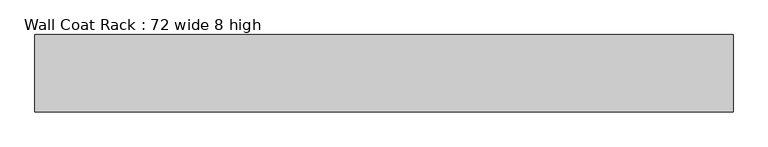
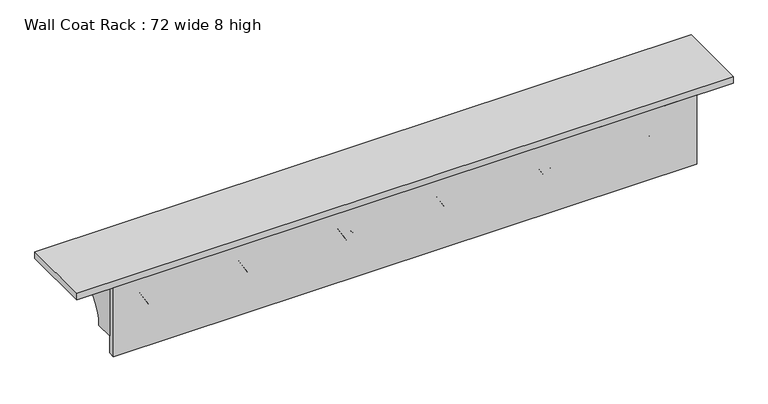
"""IFC4 building model written with IfcOpenShell, lengths in millimetres: furniture geometry, Wall Coat Rack : 72 wide 8 high."""

from ifc_helpers import new_model, si_unit, point, frame, frame_2d, origin, place, context, project, spatial, polyline, circle_curve, ellipse_curve, trimmed, segment, composite_curve, outline, extrude, source, transform, mapped, element, save
from ifc_brep_helpers import plane_surface, revolved_surface, advanced_brep


def wall_coat_rack_72_wide_8_high_2e9e28dd(model_context):
    return source(origin(), model_context, "Body", "SolidModel", [
        advanced_brep(
        [(-419.7046589, 92.075, 1574.8), (-394.3046589, 92.075, 1574.8), (-407.0046589, 92.075, 1574.8), (-419.7046589, 193.675, 1574.8), (-394.3046589, 193.675, 1574.8), (-407.0046589, 193.675, 1574.8)],
        [
            (0, 1, circle_curve(frame((-407.0046589, 92.075, 1574.8), z_axis=(0.0, -1.0, 0.0), x_axis=(1.0, 0.0, 0.0)), 12.7)),
            (1, 2),
            (2, 0),
            (1, 0, circle_curve(frame((-407.0046589, 92.075, 1574.8), z_axis=(0.0, -1.0, 0.0), x_axis=(1.0, 0.0, 0.0)), 12.7)),
            (3, 4, circle_curve(frame((-407.0046589, 193.675, 1574.8), z_axis=(0.0, -1.0, 0.0), x_axis=(1.0, 0.0, 0.0)), 12.7)),
            (4, 1, circle_curve(frame((-119.5616517, 142.875, 1574.8), z_axis=(0.0, 0.0, 1.0), x_axis=(1.0, 0.0, 0.0)), 279.4)),
            (0, 3, circle_curve(frame((-694.4476661, 142.875, 1574.8), z_axis=(0.0, 0.0, 1.0), x_axis=(-1.0, 0.0, 0.0)), 279.4)),
            (4, 3, circle_curve(frame((-407.0046589, 193.675, 1574.8), z_axis=(0.0, -1.0, 0.0), x_axis=(1.0, 0.0, 0.0)), 12.7)),
            (5, 4),
            (3, 5),
        ],
        [
            plane_surface(frame((-407.0046589, 92.075, 1574.8), z_axis=(0.0, -1.0, 0.0), x_axis=(1.0, 0.0, 0.0))),
            revolved_surface(trimmed(ellipse_curve(frame((-119.5616517, 142.875, 1574.8), z_axis=(0.0, 0.0, -1.0), x_axis=(1.0, 0.0, 0.0)), 279.4, 279.4), [point((-394.3046589, 92.075, 1574.8))], [point((-394.3046589, 193.675, 1574.8))], True, "CARTESIAN"), (-407.0046589, 193.675, 1574.8), (0.0, 1.0, 0.0)),
            plane_surface(frame((-407.0046589, 193.675, 1574.8), z_axis=(0.0, 1.0, 0.0), x_axis=(1.0, 0.0, 0.0))),
        ],
        [
            (0, [[1, 2, 3]]),
            (0, [[4, -3, -2]]),
            (1, [[5, 6, -1, 7]]),
            (1, [[8, -7, -4, -6]]),
            (2, [[9, -5, 10]]),
            (2, [[-10, -8, -9]]),
        ],
    ),
        advanced_brep(
        [(-145.3846589, 88.9, 1574.8), (-119.9846589, 88.9, 1574.8), (-132.6846589, 88.9, 1574.8), (-145.3846589, 190.5, 1574.8), (-119.9846589, 190.5, 1574.8), (-132.6846589, 190.5, 1574.8)],
        [
            (0, 1, circle_curve(frame((-132.6846589, 88.9, 1574.8), z_axis=(0.0, -1.0, 0.0), x_axis=(1.0, 0.0, 0.0)), 12.7)),
            (1, 2),
            (2, 0),
            (1, 0, circle_curve(frame((-132.6846589, 88.9, 1574.8), z_axis=(0.0, -1.0, 0.0), x_axis=(1.0, 0.0, 0.0)), 12.7)),
            (3, 4, circle_curve(frame((-132.6846589, 190.5, 1574.8), z_axis=(0.0, -1.0, 0.0), x_axis=(1.0, 0.0, 0.0)), 12.7)),
            (4, 1, circle_curve(frame((154.7583483, 139.7, 1574.8), z_axis=(0.0, 0.0, 1.0), x_axis=(1.0, 0.0, 0.0)), 279.4)),
            (0, 3, circle_curve(frame((-420.1276661, 139.7, 1574.8), z_axis=(0.0, 0.0, 1.0), x_axis=(-1.0, 0.0, 0.0)), 279.4)),
            (4, 3, circle_curve(frame((-132.6846589, 190.5, 1574.8), z_axis=(0.0, -1.0, 0.0), x_axis=(1.0, 0.0, 0.0)), 12.7)),
            (5, 4),
            (3, 5),
        ],
        [
            plane_surface(frame((-132.6846589, 88.9, 1574.8), z_axis=(0.0, -1.0, 0.0), x_axis=(1.0, 0.0, 0.0))),
            revolved_surface(trimmed(ellipse_curve(frame((154.7583483, 139.7, 1574.8), z_axis=(0.0, 0.0, -1.0), x_axis=(1.0, 0.0, 0.0)), 279.4, 279.4), [point((-119.9846589, 88.9, 1574.8))], [point((-119.9846589, 190.5, 1574.8))], True, "CARTESIAN"), (-132.6846589, 190.5, 1574.8), (0.0, 1.0, 0.0)),
            plane_surface(frame((-132.6846589, 190.5, 1574.8), z_axis=(0.0, 1.0, 0.0), x_axis=(1.0, 0.0, 0.0))),
        ],
        [
            (0, [[1, 2, 3]]),
            (0, [[4, -3, -2]]),
            (1, [[5, 6, -1, 7]]),
            (1, [[8, -7, -4, -6]]),
            (2, [[9, -5, 10]]),
            (2, [[-10, -8, -9]]),
        ],
    ),
        advanced_brep(
        [(128.9353411, 85.725, 1574.8), (154.3353411, 85.725, 1574.8), (141.6353411, 85.725, 1574.8), (128.9353411, 187.325, 1574.8), (154.3353411, 187.325, 1574.8), (141.6353411, 187.325, 1574.8)],
        [
            (0, 1, circle_curve(frame((141.6353411, 85.725, 1574.8), z_axis=(0.0, -1.0, 0.0), x_axis=(1.0, 0.0, 0.0)), 12.7)),
            (1, 2),
            (2, 0),
            (1, 0, circle_curve(frame((141.6353411, 85.725, 1574.8), z_axis=(0.0, -1.0, 0.0), x_axis=(1.0, 0.0, 0.0)), 12.7)),
            (3, 4, circle_curve(frame((141.6353411, 187.325, 1574.8), z_axis=(0.0, -1.0, 0.0), x_axis=(1.0, 0.0, 0.0)), 12.7)),
            (4, 1, circle_curve(frame((429.0783483, 136.525, 1574.8), z_axis=(0.0, 0.0, 1.0), x_axis=(1.0, 0.0, 0.0)), 279.4)),
            (0, 3, circle_curve(frame((-145.8076661, 136.525, 1574.8), z_axis=(0.0, 0.0, 1.0), x_axis=(-1.0, 0.0, 0.0)), 279.4)),
            (4, 3, circle_curve(frame((141.6353411, 187.325, 1574.8), z_axis=(0.0, -1.0, 0.0), x_axis=(1.0, 0.0, 0.0)), 12.7)),
            (5, 4),
            (3, 5),
        ],
        [
            plane_surface(frame((141.6353411, 85.725, 1574.8), z_axis=(0.0, -1.0, 0.0), x_axis=(1.0, 0.0, 0.0))),
            revolved_surface(trimmed(ellipse_curve(frame((429.0783483, 136.525, 1574.8), z_axis=(0.0, 0.0, -1.0), x_axis=(1.0, 0.0, 0.0)), 279.4, 279.4), [point((154.3353411, 85.725, 1574.8))], [point((154.3353411, 187.325, 1574.8))], True, "CARTESIAN"), (141.6353411, 187.325, 1574.8), (0.0, 1.0, 0.0)),
            plane_surface(frame((141.6353411, 187.325, 1574.8), z_axis=(0.0, 1.0, 0.0), x_axis=(1.0, 0.0, 0.0))),
        ],
        [
            (0, [[1, 2, 3]]),
            (0, [[4, -3, -2]]),
            (1, [[5, 6, -1, 7]]),
            (1, [[8, -7, -4, -6]]),
            (2, [[9, -5, 10]]),
            (2, [[-10, -8, -9]]),
        ],
    ),
        advanced_brep(
        [(403.2553411, 82.55, 1574.8), (428.6553411, 82.55, 1574.8), (415.9553411, 82.55, 1574.8), (403.2553411, 184.15, 1574.8), (428.6553411, 184.15, 1574.8), (415.9553411, 184.15, 1574.8)],
        [
            (0, 1, circle_curve(frame((415.9553411, 82.55, 1574.8), z_axis=(0.0, -1.0, 0.0), x_axis=(1.0, 0.0, 0.0)), 12.7)),
            (1, 2),
            (2, 0),
            (1, 0, circle_curve(frame((415.9553411, 82.55, 1574.8), z_axis=(0.0, -1.0, 0.0), x_axis=(1.0, 0.0, 0.0)), 12.7)),
            (3, 4, circle_curve(frame((415.9553411, 184.15, 1574.8), z_axis=(0.0, -1.0, 0.0), x_axis=(1.0, 0.0, 0.0)), 12.7)),
            (4, 1, circle_curve(frame((703.3983483, 133.35, 1574.8), z_axis=(0.0, 0.0, 1.0), x_axis=(1.0, 0.0, 0.0)), 279.4)),
            (0, 3, circle_curve(frame((128.5123339, 133.35, 1574.8), z_axis=(0.0, 0.0, 1.0), x_axis=(-1.0, 0.0, 0.0)), 279.4)),
            (4, 3, circle_curve(frame((415.9553411, 184.15, 1574.8), z_axis=(0.0, -1.0, 0.0), x_axis=(1.0, 0.0, 0.0)), 12.7)),
            (5, 4),
            (3, 5),
        ],
        [
            plane_surface(frame((415.9553411, 82.55, 1574.8), z_axis=(0.0, -1.0, 0.0), x_axis=(1.0, 0.0, 0.0))),
            revolved_surface(trimmed(ellipse_curve(frame((703.3983483, 133.35, 1574.8), z_axis=(0.0, 0.0, -1.0), x_axis=(1.0, 0.0, 0.0)), 279.4, 279.4), [point((428.6553411, 82.55, 1574.8))], [point((428.6553411, 184.15, 1574.8))], True, "CARTESIAN"), (415.9553411, 184.15, 1574.8), (0.0, 1.0, 0.0)),
            plane_surface(frame((415.9553411, 184.15, 1574.8), z_axis=(0.0, 1.0, 0.0), x_axis=(1.0, 0.0, 0.0))),
        ],
        [
            (0, [[1, 2, 3]]),
            (0, [[4, -3, -2]]),
            (1, [[5, 6, -1, 7]]),
            (1, [[8, -7, -4, -6]]),
            (2, [[9, -5, 10]]),
            (2, [[-10, -8, -9]]),
        ],
    ),
        advanced_brep(
        [(-694.0246589, 95.25, 1574.8), (-668.6246589, 95.25, 1574.8), (-681.3246589, 95.25, 1574.8), (-694.0246589, 196.85, 1574.8), (-668.6246589, 196.85, 1574.8), (-681.3246589, 196.85, 1574.8)],
        [
            (0, 1, circle_curve(frame((-681.3246589, 95.25, 1574.8), z_axis=(0.0, -1.0, 0.0), x_axis=(1.0, 0.0, 0.0)), 12.7)),
            (1, 2),
            (2, 0),
            (1, 0, circle_curve(frame((-681.3246589, 95.25, 1574.8), z_axis=(0.0, -1.0, 0.0), x_axis=(1.0, 0.0, 0.0)), 12.7)),
            (3, 4, circle_curve(frame((-681.3246589, 196.85, 1574.8), z_axis=(0.0, -1.0, 0.0), x_axis=(1.0, 0.0, 0.0)), 12.7)),
            (4, 1, circle_curve(frame((-393.8816517, 146.05, 1574.8), z_axis=(0.0, 0.0, 1.0), x_axis=(1.0, 0.0, 0.0)), 279.4)),
            (0, 3, circle_curve(frame((-968.7676661, 146.05, 1574.8), z_axis=(0.0, 0.0, 1.0), x_axis=(-1.0, 0.0, 0.0)), 279.4)),
            (4, 3, circle_curve(frame((-681.3246589, 196.85, 1574.8), z_axis=(0.0, -1.0, 0.0), x_axis=(1.0, 0.0, 0.0)), 12.7)),
            (5, 4),
            (3, 5),
        ],
        [
            plane_surface(frame((-681.3246589, 95.25, 1574.8), z_axis=(0.0, -1.0, 0.0), x_axis=(1.0, 0.0, 0.0))),
            revolved_surface(trimmed(ellipse_curve(frame((-393.8816517, 146.05, 1574.8), z_axis=(0.0, 0.0, -1.0), x_axis=(1.0, 0.0, 0.0)), 279.4, 279.4), [point((-668.6246589, 95.25, 1574.8))], [point((-668.6246589, 196.85, 1574.8))], True, "CARTESIAN"), (-681.3246589, 196.85, 1574.8), (0.0, 1.0, 0.0)),
            plane_surface(frame((-681.3246589, 196.85, 1574.8), z_axis=(0.0, 1.0, 0.0), x_axis=(1.0, 0.0, 0.0))),
        ],
        [
            (0, [[1, 2, 3]]),
            (0, [[4, -3, -2]]),
            (1, [[5, 6, -1, 7]]),
            (1, [[8, -7, -4, -6]]),
            (2, [[9, -5, 10]]),
            (2, [[-10, -8, -9]]),
        ],
    ),
        advanced_brep(
        [(677.5753411, 79.375, 1574.8), (702.9753411, 79.375, 1574.8), (690.2753411, 79.375, 1574.8), (677.5753411, 180.975, 1574.8), (702.9753411, 180.975, 1574.8), (690.2753411, 180.975, 1574.8)],
        [
            (0, 1, circle_curve(frame((690.2753411, 79.375, 1574.8), z_axis=(0.0, -1.0, 0.0), x_axis=(1.0, 0.0, 0.0)), 12.7)),
            (1, 2),
            (2, 0),
            (1, 0, circle_curve(frame((690.2753411, 79.375, 1574.8), z_axis=(0.0, -1.0, 0.0), x_axis=(1.0, 0.0, 0.0)), 12.7)),
            (3, 4, circle_curve(frame((690.2753411, 180.975, 1574.8), z_axis=(0.0, -1.0, 0.0), x_axis=(1.0, 0.0, 0.0)), 12.7)),
            (4, 1, circle_curve(frame((977.7183483, 130.175, 1574.8), z_axis=(0.0, 0.0, 1.0), x_axis=(1.0, 0.0, 0.0)), 279.4)),
            (0, 3, circle_curve(frame((402.8323339, 130.175, 1574.8), z_axis=(0.0, 0.0, 1.0), x_axis=(-1.0, 0.0, 0.0)), 279.4)),
            (4, 3, circle_curve(frame((690.2753411, 180.975, 1574.8), z_axis=(0.0, -1.0, 0.0), x_axis=(1.0, 0.0, 0.0)), 12.7)),
            (5, 4),
            (3, 5),
        ],
        [
            plane_surface(frame((690.2753411, 79.375, 1574.8), z_axis=(0.0, -1.0, 0.0), x_axis=(1.0, 0.0, 0.0))),
            revolved_surface(trimmed(ellipse_curve(frame((977.7183483, 130.175, 1574.8), z_axis=(0.0, 0.0, -1.0), x_axis=(1.0, 0.0, 0.0)), 279.4, 279.4), [point((702.9753411, 79.375, 1574.8))], [point((702.9753411, 180.975, 1574.8))], True, "CARTESIAN"), (690.2753411, 180.975, 1574.8), (0.0, 1.0, 0.0)),
            plane_surface(frame((690.2753411, 180.975, 1574.8), z_axis=(0.0, 1.0, 0.0), x_axis=(1.0, 0.0, 0.0))),
        ],
        [
            (0, [[1, 2, 3]]),
            (0, [[4, -3, -2]]),
            (1, [[5, 6, -1, 7]]),
            (1, [[8, -7, -4, -6]]),
            (2, [[9, -5, 10]]),
            (2, [[-10, -8, -9]]),
        ],
    ),
        extrude(outline(composite_curve([segment(polyline([(231.775, 1676.4), (231.775, 1625.6)]), True, "CONTINUOUS"), segment(trimmed(circle_curve(frame_2d((231.775, 1524.0)), 101.6), [point((231.775, 1625.6))], [point((130.175, 1524.0))], True, "CARTESIAN"), True, "CONTINUOUS"), segment(polyline([(130.175, 1524.0), (79.375, 1524.0), (79.375, 1676.4), (231.775, 1676.4)]), True, "CONTINUOUS")], self_intersect=False)), frame((-808.3246589, 0.0, 0.0), z_axis=(1.0, 0.0, 0.0), x_axis=(0.0, 1.0, 0.0)), (0.0, 0.0, 1.0), 19.05),
        extrude(outline(composite_curve([segment(polyline([(231.775, 1676.4), (231.775, 1625.6)]), True, "CONTINUOUS"), segment(trimmed(circle_curve(frame_2d((231.775, 1524.0)), 101.6), [point((231.775, 1625.6))], [point((130.175, 1524.0))], True, "CARTESIAN"), True, "CONTINUOUS"), segment(polyline([(130.175, 1524.0), (79.375, 1524.0), (79.375, 1676.4), (231.775, 1676.4)]), True, "CONTINUOUS")], self_intersect=False)), frame((798.2253411, 0.0, 0.0), z_axis=(1.0, 0.0, 0.0), x_axis=(0.0, 1.0, 0.0)), (0.0, 0.0, 1.0), 19.05),
        extrude(outline(polyline([(-808.3246589, 79.375), (817.2753411, 79.375), (817.2753411, 60.325), (-808.3246589, 60.325), (-808.3246589, 79.375)])), frame((0.0, 0.0, 1473.2), z_axis=(0.0, 0.0, 1.0), x_axis=(1.0, 0.0, 0.0)), (0.0, 0.0, 1.0), 203.2),
        extrude(outline(polyline([(918.8753411, 60.325), (-909.9246589, 60.325), (-909.9246589, 263.525), (918.8753411, 263.525), (918.8753411, 60.325)])), frame((0.0, 0.0, 1676.4), z_axis=(0.0, 0.0, 1.0), x_axis=(1.0, 0.0, 0.0)), (0.0, 0.0, 1.0), 19.05),
    ])


if __name__ == "__main__":
    model = new_model("IFC4")
    model_context = context("Model", 3, world=origin())
    ifc_project = project(units=[si_unit("LENGTHUNIT", "METRE", prefix="MILLI")], contexts=[model_context])
    site = spatial("IfcSite", under=ifc_project)
    building = spatial("IfcBuilding", under=site)
    placement = place(None, origin())
    wall_coat_rack_72_wide_8_high_shape = wall_coat_rack_72_wide_8_high_2e9e28dd(model_context)
    element("IfcFurniture", 1, ObjectType="Wall Coat Rack : 72 wide 8 high", at=placement, inside=building, context=model_context, shape_type="MappedRepresentation", body=[
        mapped(wall_coat_rack_72_wide_8_high_shape, transform((0.0, 0.0, 0.0), x_axis=(1.0, 0.0, 0.0), y_axis=(0.0, 1.0, 0.0), z_axis=(0.0, 0.0, 1.0))),
    ])
    save(model, "model.ifc")

# Revit data of these elements
# Type "Wall Coat Rack : 72 wide 8 high"
#   Width = 6' - 0"
#   Mounting Height = 5' - 6"
#   Hook Inset = 0' - 5"
#   Hook Height = 5' - 2"
#   Height = 0' - 8"
#   Show Hook = yes
#   Number of Hooks = 6
#   Shelf and Backing [instance default] = none
#   Hook [instance default] = none
#   Default Elevation = 0
# Element 1 (IfcFurniture, "Wall Coat Rack : 72 wide 8 high")
#   Shelf and Backing = Maple - Semigloss(Rotated)
#   Hook = Maple - Semigloss
#   Materials on its faces: "Maple - Semigloss", "Maple - Semigloss(Rotated)"
# Materials
#   "Maple - Semigloss": class "Wood", colour RGB 196 161 118, transparency 0, Description = "Acer Saccharum", Cost = 0
#   "Maple - Semigloss(Rotated)": class "Wood", colour RGB 196 161 118, transparency 0, Description = "Acer Saccharum", Cost = 0
